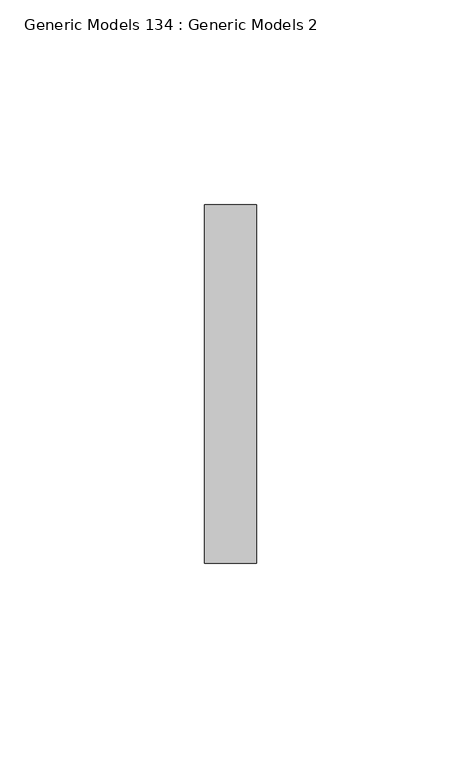
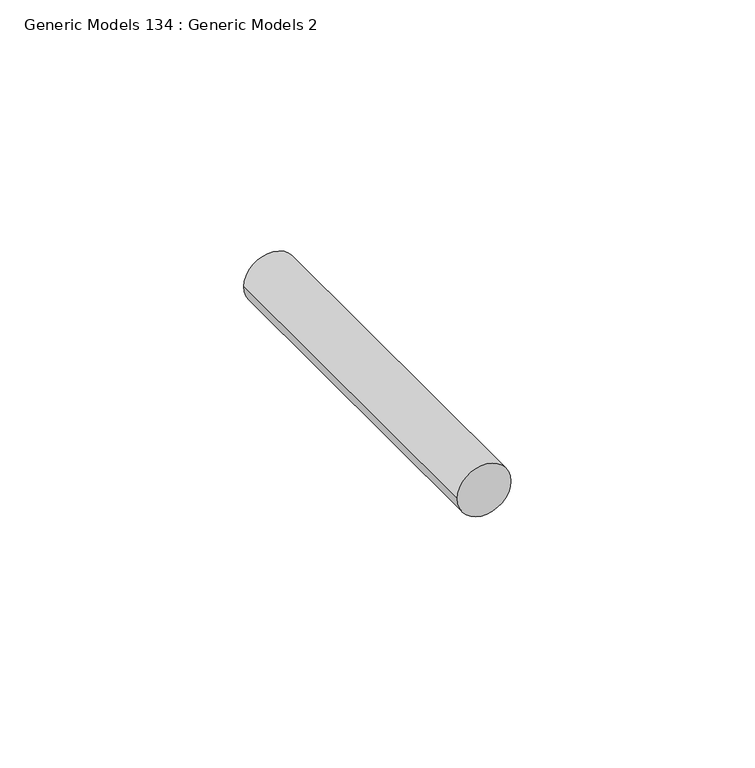
"""IFC4 building model written with IfcOpenShell, lengths in millimetres: proxy geometry, Generic Models 134 : Generic Models 2."""

from ifc_helpers import new_model, si_unit, point, frame, frame_2d, origin, place, context, project, spatial, circle_curve, trimmed, segment, composite_curve, outline, extrude, source, transform, mapped, element, save


def generic_models_134_generic_models_2_8934cadc(model_context):
    return source(origin(), model_context, "Body", "SweptSolid", [
        extrude(outline(composite_curve([segment(trimmed(circle_curve(frame_2d((38717.9805939, 8245.7828124)), 6.35), [point((38717.9805939, 8239.4328124))], [point((38717.9805939, 8252.1328124))], False, "CARTESIAN"), True, "CONTINUOUS"), segment(trimmed(circle_curve(frame_2d((38717.9805939, 8245.7828124)), 6.35), [point((38717.9805939, 8252.1328124))], [point((38717.9805939, 8239.4328124))], False, "CARTESIAN"), True, "CONTINUOUS")], self_intersect=False)), frame((0.0, 1848.3666731, 0.0), z_axis=(0.0, 1.0, 0.0), x_axis=(0.0, 0.0, 1.0)), (0.0, 0.0, 1.0), 87.551022),
    ])


if __name__ == "__main__":
    model = new_model("IFC4")
    model_context = context("Model", 3, world=origin())
    ifc_project = project(units=[si_unit("LENGTHUNIT", "METRE", prefix="MILLI")], contexts=[model_context])
    site = spatial("IfcSite", under=ifc_project)
    building = spatial("IfcBuilding", under=site)
    placement = place(None, origin())
    generic_models_134_generic_models_2_shape = generic_models_134_generic_models_2_8934cadc(model_context)
    element("IfcBuildingElementProxy", 1, Name="Generic Models 134 : Generic Models 2", ObjectType="Generic Models 134 : Generic Models 2", at=placement, inside=building, context=model_context, shape_type="MappedRepresentation", body=[
        mapped(generic_models_134_generic_models_2_shape, transform((0.0, 0.0, 0.0), x_axis=(1.0, 0.0, 0.0), y_axis=(0.0, 1.0, 0.0), z_axis=(0.0, 0.0, 1.0))),
    ])
    save(model, "model.ifc")

# Revit data of these elements
# Element 1 (IfcBuildingElementProxy, "Generic Models 134 : Generic Models 2")
#   Materials on its faces: "S.S. LAG BOLT - SEE STRUCT. DWGS"
# Materials
#   "S.S. LAG BOLT - SEE STRUCT. DWGS": class "Generic", colour RGB 120 120 120, transparency 0, Cost = 0
